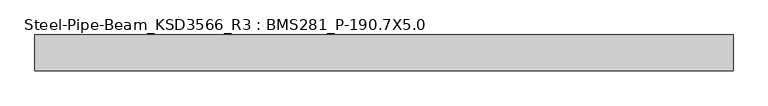
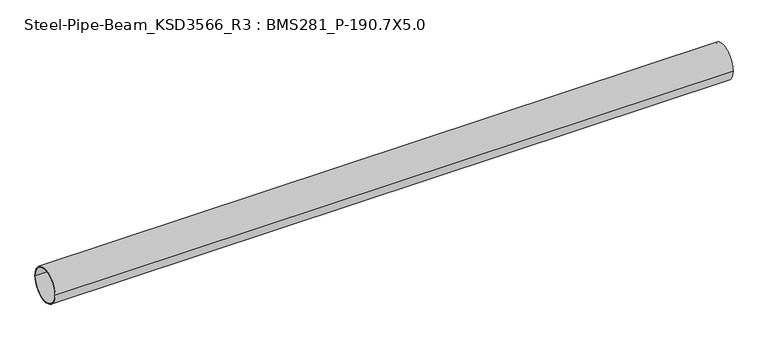
"""IFC4 building model written with IfcOpenShell, lengths in millimetres: member geometry, Steel-Pipe-Beam_KSD3566_R3 : BMS281_P-190.7X5.0."""

from ifc_helpers import new_model, si_unit, point, frame, origin, origin_2d, place, context, project, spatial, circle_curve, trimmed, segment, composite_curve, outline, extrude, source, transform, mapped, element, save


def steel_pipe_beam_ksd3566_r3_bms281_p_190_7x5_0_4d357c7a(model_context):
    return source(origin(), model_context, "Body", "SweptSolid", [
        extrude(outline(composite_curve([segment(trimmed(circle_curve(origin_2d(), 95.35), [point((-95.35, 0.0))], [point((95.35, 0.0))], False, "CARTESIAN"), True, "CONTINUOUS"), segment(trimmed(circle_curve(origin_2d(), 95.35), [point((95.35, 0.0))], [point((-95.35, 0.0))], False, "CARTESIAN"), True, "CONTINUOUS")], self_intersect=False), holes=[composite_curve([segment(trimmed(circle_curve(origin_2d(), 90.35), [point((90.35, 0.0))], [point((-90.35, 0.0))], True, "CARTESIAN"), True, "CONTINUOUS"), segment(trimmed(circle_curve(origin_2d(), 90.35), [point((-90.35, 0.0))], [point((90.35, 0.0))], True, "CARTESIAN"), True, "CONTINUOUS")], self_intersect=False)]), frame((-1840.2747831, 0.0, 0.0), z_axis=(1.0, 0.0, 0.0), x_axis=(0.0, 1.0, 0.0)), (0.0, 0.0, 1.0), 3728.144755),
    ])


if __name__ == "__main__":
    model = new_model("IFC4")
    model_context = context("Model", 3, world=origin())
    ifc_project = project(units=[si_unit("LENGTHUNIT", "METRE", prefix="MILLI")], contexts=[model_context])
    site = spatial("IfcSite", under=ifc_project)
    building = spatial("IfcBuilding", under=site)
    placement = place(None, origin())
    steel_pipe_beam_ksd3566_r3_bms281_p_190_7x5_0_shape = steel_pipe_beam_ksd3566_r3_bms281_p_190_7x5_0_4d357c7a(model_context)
    element("IfcMember", 1, ObjectType="Steel-Pipe-Beam_KSD3566_R3 : BMS281_P-190.7X5.0", at=placement, inside=building, context=model_context, shape_type="MappedRepresentation", body=[
        mapped(steel_pipe_beam_ksd3566_r3_bms281_p_190_7x5_0_shape, transform((0.0, 0.0, 0.0), x_axis=(1.0, 0.0, 0.0), y_axis=(0.0, 1.0, 0.0), z_axis=(0.0, 0.0, 1.0))),
    ])
    save(model, "model.ifc")

# Revit data of these elements
# Type "Steel-Pipe-Beam_KSD3566_R3 : BMS281_P-190.7X5.0"
#   Keynote = "P-190.7X5.0"
#   SteelWeight = "Light"
#   t = 0.0050 m
#   Surface Area = 0.599102 m²/m
#   Section Area = 29.1697 cm²
#   Mass per Unit Length = 22.8982 kg/m
#   Length [instance default] = 1.5000 m
#   D = 0.1907 m
#   hec_material4 [instance default] = none
#   hec_material3 [instance default] = none
#   hec_material2 [instance default] = none
#   hec_material1 [instance default] = none
#   Structural Material [instance default] = Steel, 45-345
#   Assembly Code = ""
# Element 1 (IfcMember, "Steel-Pipe-Beam_KSD3566_R3 : BMS281_P-190.7X5.0")
#   Structural Material = none
# Materials
#   "Steel, 45-345": class "Metal", colour RGB 189 187 185, transparency 0, Description = "Steel 345 MPa", Cost = 0
